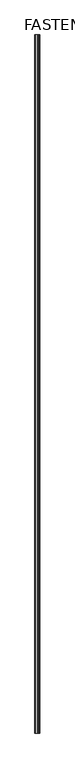
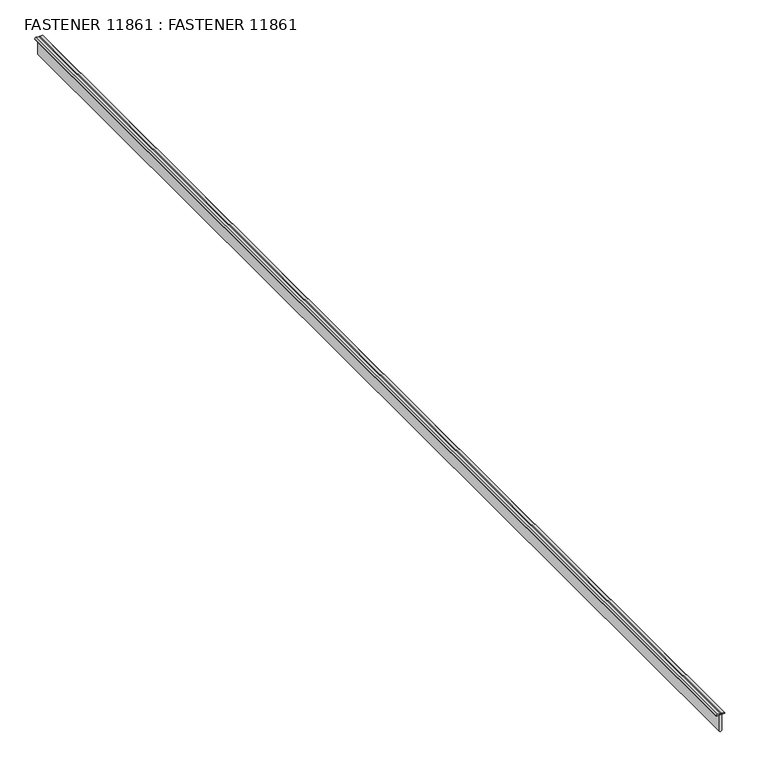
"""IFC4 building model written with IfcOpenShell, lengths in millimetres: proxy geometry, FASTENER 11861 : FASTENER 11861."""

from ifc_helpers import new_model, si_unit, frame, origin, place, context, project, spatial, polyline, outline, extrude, source, transform, mapped, element, save


def fastener_11861_fastener_11861_40db04d7(model_context):
    return source(origin(), model_context, "Body", "SweptSolid", [
        extrude(outline(polyline([(42551.3049701, 5981.517626), (42579.6987049, 5981.517626), (42579.6987049, 5977.3107075), (42550.7399648, 5977.3107075), (42549.1244121, 5978.9677221), (42551.3049701, 5981.517626)])), frame((0.0, -1052.8906574, 0.0), z_axis=(0.0, 1.0, 0.0), x_axis=(0.0, 0.0, 1.0)), (0.0, 0.0, 1.0), 1999.85),
        extrude(outline(polyline([(42580.5349921, 5972.2779845), (42579.6987049, 5972.2671879), (42579.6987049, 5986.5634932), (42580.508527, 5986.5634932), (42582.1023984, 5985.3247911), (42582.1023984, 5980.4457092), (42580.1167322, 5980.0391089), (42580.1167322, 5978.792004), (42581.7222633, 5978.792004), (42582.1288635, 5973.5166866), (42580.5349921, 5972.2779845)])), frame((0.0, -1052.8906574, 0.0), z_axis=(0.0, 1.0, 0.0), x_axis=(0.0, 0.0, 1.0)), (0.0, 0.0, 1.0), 1999.85),
    ])


if __name__ == "__main__":
    model = new_model("IFC4")
    model_context = context("Model", 3, world=origin())
    ifc_project = project(units=[si_unit("LENGTHUNIT", "METRE", prefix="MILLI")], contexts=[model_context])
    site = spatial("IfcSite", under=ifc_project)
    building = spatial("IfcBuilding", under=site)
    placement = place(None, origin())
    fastener_11861_fastener_11861_shape = fastener_11861_fastener_11861_40db04d7(model_context)
    element("IfcBuildingElementProxy", 1, Name="FASTENER 11861 : FASTENER 11861", ObjectType="FASTENER 11861 : FASTENER 11861", at=placement, inside=building, context=model_context, shape_type="MappedRepresentation", body=[
        mapped(fastener_11861_fastener_11861_shape, transform((0.0, 0.0, 0.0), x_axis=(1.0, 0.0, 0.0), y_axis=(0.0, 1.0, 0.0), z_axis=(0.0, 0.0, 1.0))),
    ])
    save(model, "model.ifc")

# Revit data of these elements
# Type "FASTENER 11861 : FASTENER 11861"
#   NameOverride = "FASTENER"
# Element 1 (IfcBuildingElementProxy, "FASTENER 11861 : FASTENER 11861")
#   Materials on its faces: "ENGINEERED PANCAKE HEAD FASTENER @ 12\" O.C."
# Materials
#   "ENGINEERED PANCAKE HEAD FASTENER @ 12\" O.C.": class "Unassigned", colour RGB 255 255 255, transparency 0, Cost = 0
